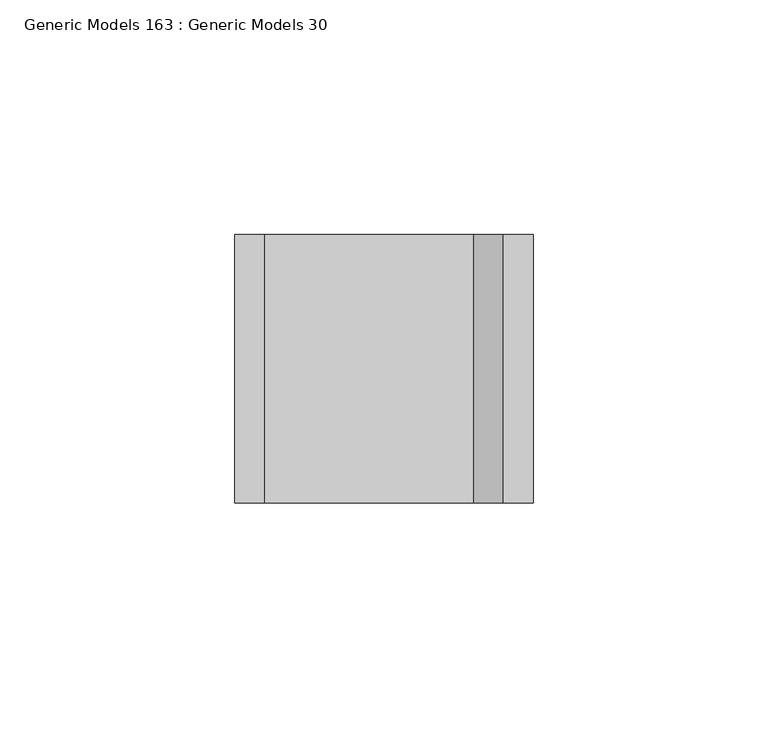
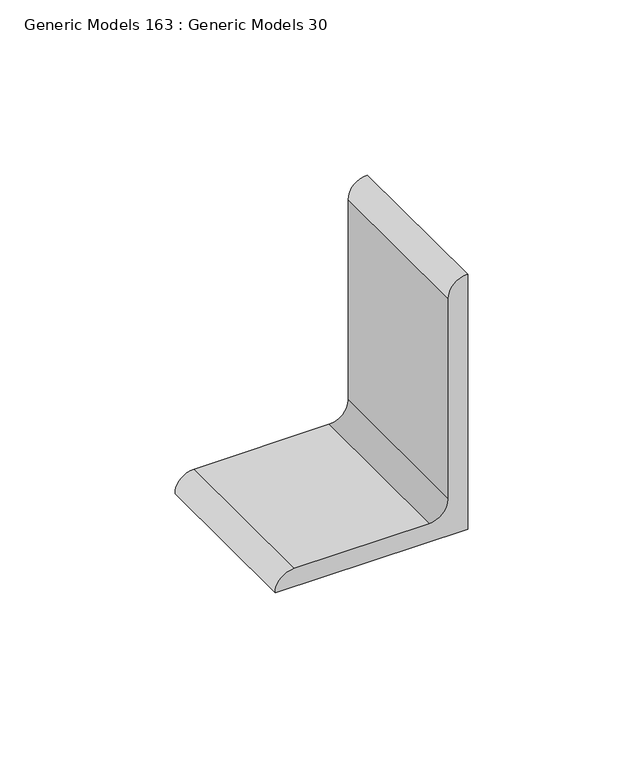
"""IFC4 building model written with IfcOpenShell, lengths in millimetres: proxy geometry, Generic Models 163 : Generic Models 30."""

from ifc_helpers import new_model, si_unit, point, frame, frame_2d, origin, place, context, project, spatial, polyline, circle_curve, trimmed, segment, composite_curve, outline, extrude, source, transform, mapped, element, save


def generic_models_163_generic_models_30_ecc5328c(model_context):
    return source(origin(), model_context, "Body", "SweptSolid", [
        extrude(outline(composite_curve([segment(polyline([(266401.55, 33370.8340778), (266490.45, 33370.8340778)]), True, "CONTINUOUS"), segment(trimmed(circle_curve(frame_2d((266484.1, 33370.8340778)), 6.35), [point((266490.45, 33370.8340778))], [point((266484.1, 33364.4840778))], False, "CARTESIAN"), True, "CONTINUOUS"), segment(polyline([(266484.1, 33364.4840778), (266414.25, 33364.4840778)]), True, "CONTINUOUS"), segment(trimmed(circle_curve(frame_2d((266414.25, 33358.1340778)), 6.35), [point((266414.25, 33364.4840778))], [point((266407.9, 33358.1340778))], True, "CARTESIAN"), True, "CONTINUOUS"), segment(polyline([(266407.9, 33358.1340778), (266407.9, 33313.6840778)]), True, "CONTINUOUS"), segment(trimmed(circle_curve(frame_2d((266401.55, 33313.6840778)), 6.35), [point((266407.9, 33313.6840778))], [point((266401.55, 33307.3340778))], False, "CARTESIAN"), True, "CONTINUOUS"), segment(polyline([(266401.55, 33307.3340778), (266401.55, 33370.8340778)]), True, "CONTINUOUS")], self_intersect=False)), frame((0.0, 41007.6196612, 0.0), z_axis=(0.0, 1.0, 0.0), x_axis=(0.0, 0.0, 1.0)), (0.0, 0.0, 1.0), 57.15),
    ])


if __name__ == "__main__":
    model = new_model("IFC4")
    model_context = context("Model", 3, world=origin())
    ifc_project = project(units=[si_unit("LENGTHUNIT", "METRE", prefix="MILLI")], contexts=[model_context])
    site = spatial("IfcSite", under=ifc_project)
    building = spatial("IfcBuilding", under=site)
    placement = place(None, origin())
    generic_models_163_generic_models_30_shape = generic_models_163_generic_models_30_ecc5328c(model_context)
    element("IfcBuildingElementProxy", 1, Name="Generic Models 163 : Generic Models 30", ObjectType="Generic Models 163 : Generic Models 30", at=placement, inside=building, context=model_context, shape_type="MappedRepresentation", body=[
        mapped(generic_models_163_generic_models_30_shape, transform((0.0, 0.0, 0.0), x_axis=(1.0, 0.0, 0.0), y_axis=(0.0, 1.0, 0.0), z_axis=(0.0, 0.0, 1.0))),
    ])
    save(model, "model.ifc")

# Revit data of these elements
# Element 1 (IfcBuildingElementProxy, "Generic Models 163 : Generic Models 30")
#   Materials on its faces: "GALV 3 1/2\"X 2 1/2\" X 1/4\" STEEL ANGLE - WELD TO VERTICAL STEEL ANGLE"
# Materials
#   "GALV 3 1/2\"X 2 1/2\" X 1/4\" STEEL ANGLE - WELD TO VERTICAL STEEL ANGLE": class "Metal", colour RGB 199 199 199, transparency 0, Description = "Structural steel, ASTM A36 Grade B, mill finish", Cost = 0
